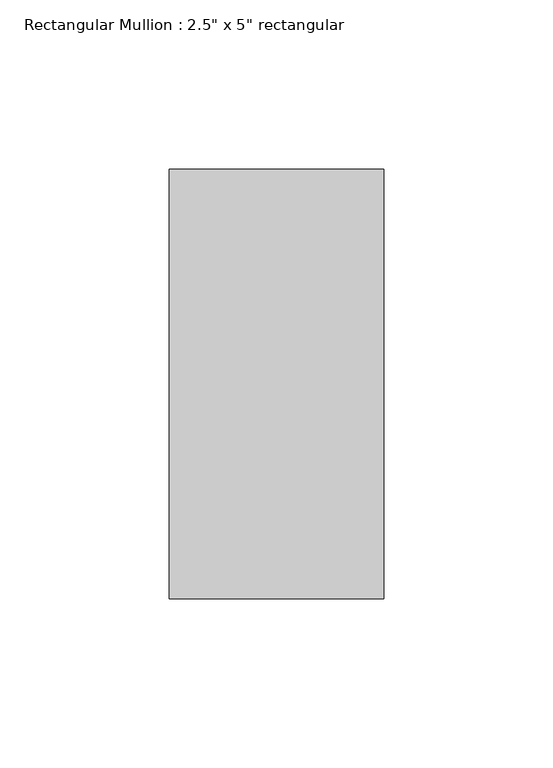
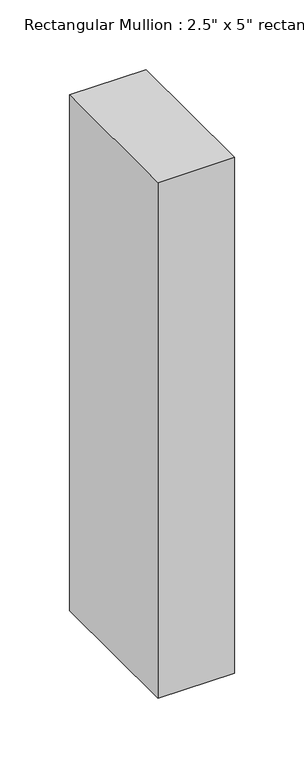
"""IFC4 building model written with IfcOpenShell, lengths in millimetres: member geometry."""

from ifc_helpers import new_model, si_unit, frame, origin, place, context, project, spatial, polyline, outline, extrude, source, transform, mapped, element, save


def member_210120dd(model_context):
    return source(origin(), model_context, "Body", "SweptSolid", [
        extrude(outline(polyline([(31.75, 63.5), (31.75, -63.5), (-31.75, -63.5), (-31.75, 63.5), (31.75, 63.5)])), frame((0.0, 0.0, -451.964047), z_axis=(0.0, 0.0, 1.0), x_axis=(1.0, 0.0, 0.0)), (0.0, 0.0, 1.0), 451.964047),
    ])


if __name__ == "__main__":
    model = new_model("IFC4")
    model_context = context("Model", 3, world=origin())
    ifc_project = project(units=[si_unit("LENGTHUNIT", "METRE", prefix="MILLI")], contexts=[model_context])
    site = spatial("IfcSite", under=ifc_project)
    building = spatial("IfcBuilding", under=site)
    placement = place(None, origin())
    member_shape = member_210120dd(model_context)
    element("IfcMember", 1, ObjectType="Rectangular Mullion : 2.5\" x 5\" rectangular", at=placement, inside=building, context=model_context, shape_type="MappedRepresentation", body=[
        mapped(member_shape, transform((0.0, 0.0, 0.0), x_axis=(1.0, 0.0, 0.0), y_axis=(0.0, 1.0, 0.0), z_axis=(0.0, 0.0, 1.0))),
    ])
    save(model, "model.ifc")

# Revit data of these elements
# Type "Rectangular Mullion : 2.5\" x 5\" rectangular"
#   built-in parameter 1007304 = 0.416667 (stored number, unit not read)
#   built-in parameter 1007301 = 0.104167 (stored number, unit not read)
#   built-in parameter 1007300 = 0.104167 (stored number, unit not read)
# Element 1 (IfcMember, "Rectangular Mullion : 2.5\" x 5\" rectangular")
#   Materials on its faces: "Metal - Aluminum 2"
# Materials
#   "Metal - Aluminum 2": class "Metal", colour RGB 189 187 185, transparency 0
